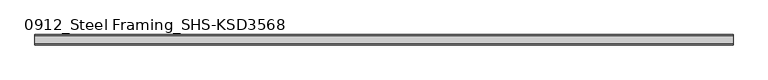
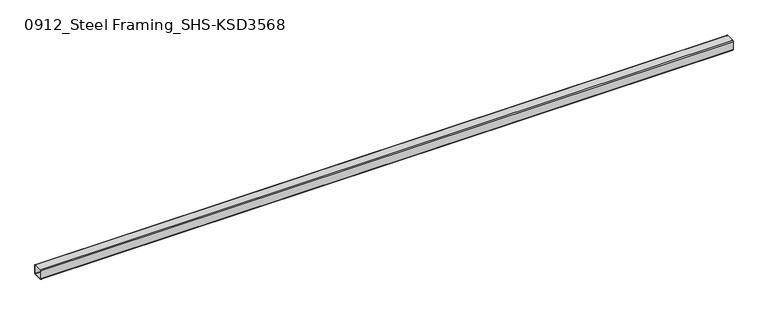
"""IFC4 building model written with IfcOpenShell, lengths in millimetres: beam geometry, 0912_Steel Framing_SHS-KSD3568 : H_SB_ASB_SHS-150x150x6."""

from ifc_helpers import new_model, si_unit, point, frame, frame_2d, origin, place, context, project, spatial, polyline, circle_curve, trimmed, segment, composite_curve, outline, extrude, source, transform, mapped, element, save


def beam_0912_steel_framing_shs_ksd3568_59c60497(model_context):
    return source(origin(), model_context, "Body", "SweptSolid", [
        extrude(outline(composite_curve([segment(polyline([(75.0, 63.0), (75.0, -63.0)]), True, "CONTINUOUS"), segment(trimmed(circle_curve(frame_2d((63.0, -63.0)), 12.0), [point((75.0, -63.0))], [point((63.0, -75.0))], False, "CARTESIAN"), True, "CONTINUOUS"), segment(polyline([(63.0, -75.0), (-63.0, -75.0)]), True, "CONTINUOUS"), segment(trimmed(circle_curve(frame_2d((-63.0, -63.0)), 12.0), [point((-63.0, -75.0))], [point((-75.0, -63.0))], False, "CARTESIAN"), True, "CONTINUOUS"), segment(polyline([(-75.0, -63.0), (-75.0, 63.0)]), True, "CONTINUOUS"), segment(trimmed(circle_curve(frame_2d((-63.0, 63.0)), 12.0), [point((-75.0, 63.0))], [point((-63.0, 75.0))], False, "CARTESIAN"), True, "CONTINUOUS"), segment(polyline([(-63.0, 75.0), (63.0, 75.0)]), True, "CONTINUOUS"), segment(trimmed(circle_curve(frame_2d((63.0, 63.0)), 12.0), [point((63.0, 75.0))], [point((75.0, 63.0))], False, "CARTESIAN"), True, "CONTINUOUS")], self_intersect=False), holes=[composite_curve([segment(trimmed(circle_curve(frame_2d((-63.0, 63.0)), 6.0), [point((-63.0, 69.0))], [point((-69.0, 63.0))], True, "CARTESIAN"), True, "CONTINUOUS"), segment(polyline([(-69.0, 63.0), (-69.0, -63.0)]), True, "CONTINUOUS"), segment(trimmed(circle_curve(frame_2d((-63.0, -63.0)), 6.0), [point((-69.0, -63.0))], [point((-63.0, -69.0))], True, "CARTESIAN"), True, "CONTINUOUS"), segment(polyline([(-63.0, -69.0), (63.0, -69.0)]), True, "CONTINUOUS"), segment(trimmed(circle_curve(frame_2d((63.0, -63.0)), 6.0), [point((63.0, -69.0))], [point((69.0, -63.0))], True, "CARTESIAN"), True, "CONTINUOUS"), segment(polyline([(69.0, -63.0), (69.0, 63.0)]), True, "CONTINUOUS"), segment(trimmed(circle_curve(frame_2d((63.0, 63.0)), 6.0), [point((69.0, 63.0))], [point((63.0, 69.0))], True, "CARTESIAN"), True, "CONTINUOUS"), segment(polyline([(63.0, 69.0), (-63.0, 69.0)]), True, "CONTINUOUS")], self_intersect=False)]), frame((-5049.8, 0.0, 0.0), z_axis=(1.0, 0.0, 0.0), x_axis=(0.0, 1.0, 0.0)), (0.0, 0.0, 1.0), 10224.6),
    ])


if __name__ == "__main__":
    model = new_model("IFC4")
    model_context = context("Model", 3, world=origin())
    ifc_project = project(units=[si_unit("LENGTHUNIT", "METRE", prefix="MILLI")], contexts=[model_context])
    site = spatial("IfcSite", under=ifc_project)
    building = spatial("IfcBuilding", under=site)
    placement = place(None, origin())
    beam_0912_steel_framing_shs_ksd3568_shape = beam_0912_steel_framing_shs_ksd3568_59c60497(model_context)
    element("IfcBeam", 1, ObjectType="0912_Steel Framing_SHS-KSD3568 : H_SB_ASB_SHS-150x150x6", at=placement, inside=building, context=model_context, shape_type="MappedRepresentation", body=[
        mapped(beam_0912_steel_framing_shs_ksd3568_shape, transform((0.0, 0.0, 0.0), x_axis=(1.0, 0.0, 0.0), y_axis=(0.0, 1.0, 0.0), z_axis=(0.0, 0.0, 1.0))),
    ])
    save(model, "model.ifc")

# Revit data of these elements
# Type "0912_Steel Framing_SHS-KSD3568 : H_SB_ASB_SHS-150x150x6"
#   H_WM Code_1 = "S01AA002-00001 | Main Steel Structure Fabrication Work | Shelter/Building | Medium Steel - Standard (90KG/M>Weight≥30KG/M) | Material: (   )"
#   H_WM Code_2 = "S03AA028-00001 | Main Steel Structure Erection Work | Shelter/Building | Medium Steel (90KG/M>Weight≥30KG/M) | Material: (   )"
#   H_WM Code_3 = "S01AA010-00001 | Main Steel Structure Fabrication Work | Shelter/Building | Steel Painting/Coating | for Non-Fireproofed Steel Surface, Surface Preparation, Primer, Second & Final Coat | Material: (   )"
#   H_Q'ty Cal Type Tag = "SB-Q2"
#   Perimeter = 0.60 m²/m
#   Nominal Weight = 26.40 kgf/m
#   Length [instance default] = 1.0000 m
#   b = 0.1500 m
#   h = 0.1500 m
#   tr = 0.0120 m
#   t = 0.0060 m
#   A = 28.36 m²
#   Structural Material [instance default] = Steel, 45-345
# Element 1 (IfcBeam, "0912_Steel Framing_SHS-KSD3568 : H_SB_ASB_SHS-150x150x6")
#   Structural Material = none
# Materials
#   "Steel, 45-345": class "Metal", colour RGB 189 187 185, transparency 0, Description = "Steel 345 MPa", Cost = 0
